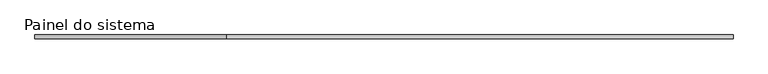
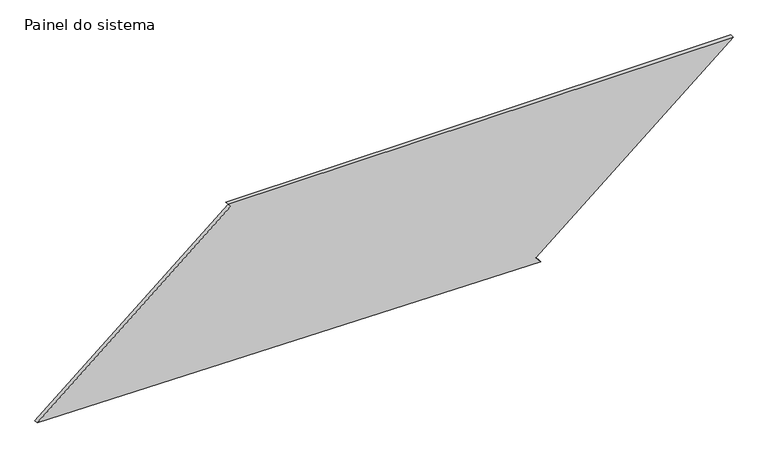
"""IFC4 building model written with IfcOpenShell, lengths in millimetres: plate geometry, Painel do sistema : Envidraçado."""

import ifcopenshell
import ifcopenshell.guid

model = None  # the IFC model being written
_history = None  # IfcOwnerHistory: only IFC2X3 demands one
_inside = {}  # id of a spatial element -> (the spatial element, [elements in it])
_under = {}  # id of a project, library or spatial element -> (it, [spatial elements below it])
_declared = {}  # id of a project -> (the project, [libraries it declares])
_typed = {}  # id of a type object -> (the type object, [elements of that type])
_made_of = {}  # id of a material, layer set ... -> (it, [elements and type objects made of it])


def new_model(schema):
    """Start an empty IFC model of exactly this schema.

    Asked for "IFC4X3", IfcOpenShell would pick the latest addendum, in which some entities
    have other attributes; the version numbers below select the first issue.
    IFC2X3 requires an IfcOwnerHistory on every rooted entity: one is made here for all.
    """
    global model, _history
    if schema == "IFC4X3":
        model = ifcopenshell.file(schema_version=(4, 3, 0, 0))
    else:
        model = ifcopenshell.file(schema=schema)
    _inside.clear()
    _under.clear()
    _declared.clear()
    _typed.clear()
    _made_of.clear()
    _history = None
    if model.schema == "IFC2X3":
        org = make("IfcOrganization", Name="unknown")
        user = make(
            "IfcPersonAndOrganization",
            ThePerson=make("IfcPerson", FamilyName="unknown"),
            TheOrganization=org,
        )
        app = make(
            "IfcApplication",
            ApplicationDeveloper=org,
            Version="unknown",
            ApplicationFullName="unknown",
            ApplicationIdentifier="unknown",
        )
        _history = make(
            "IfcOwnerHistory",
            OwningUser=user,
            OwningApplication=app,
            ChangeAction="ADDED",
            CreationDate=0,
        )
    return model


def make(cls, **values):
    """One entity of the class cls with the attributes given. An attribute that is None is left unset."""
    return model.create_entity(
        cls, **{name: value for name, value in values.items() if value is not None}
    )


def rooted(cls, **values):
    """An entity with a GlobalId (a new one), such as an element, a storey or a relation."""
    return make(cls, GlobalId=ifcopenshell.guid.new(), OwnerHistory=_history, **values)


def si_unit(unit_type, name, prefix=None):
    """IfcSIUnit, for example si_unit("LENGTHUNIT", "METRE", prefix="MILLI")."""
    return make("IfcSIUnit", UnitType=unit_type, Prefix=prefix, Name=name)


def assignment(units):
    """IfcUnitAssignment: the units of a project."""
    return None if units is None else make("IfcUnitAssignment", Units=units)


def point(xyz):
    """IfcCartesianPoint."""
    return None if xyz is None else make("IfcCartesianPoint", Coordinates=xyz)


def direction(xyz):
    """IfcDirection."""
    return None if xyz is None else make("IfcDirection", DirectionRatios=xyz)


def frame(location, z_axis=None, x_axis=None):
    """IfcAxis2Placement3D, a coordinate frame: its origin and axes. An axis left out is left unset."""
    return make(
        "IfcAxis2Placement3D",
        Location=point(location),
        Axis=direction(z_axis),
        RefDirection=direction(x_axis),
    )


def origin():
    """The frame at (0, 0, 0) with its axes left unset."""
    return frame((0.0, 0.0, 0.0))


def place(relative_to, where):
    """IfcLocalPlacement: puts the frame where relative to a parent placement (None: the world)."""
    return make(
        "IfcLocalPlacement", PlacementRelTo=relative_to, RelativePlacement=where
    )


def context(
    kind, dimensions, precision=None, world=None, true_north=None, identifier=None
):
    """IfcGeometricRepresentationContext, for example the 3D "Model" context."""
    return make(
        "IfcGeometricRepresentationContext",
        ContextIdentifier=identifier,
        ContextType=kind,
        CoordinateSpaceDimension=dimensions,
        Precision=precision,
        WorldCoordinateSystem=world,
        TrueNorth=true_north,
    )


def project(units=None, contexts=None):
    """IfcProject with its units and contexts."""
    return rooted(
        "IfcProject",
        Name="project",
        RepresentationContexts=contexts,
        UnitsInContext=assignment(units),
    )


def spatial(cls, under=None, at=None, **own):
    """A site, building, storey or space (cls), placed at a placement, below another one or the project."""
    s = rooted(cls, ObjectPlacement=at, **own)
    if under is not None:
        _under.setdefault(under.id(), (under, []))[1].append(s)
    return s


def polyline(points):
    """IfcPolyline through the points."""
    return make("IfcPolyline", Points=[point(p) for p in points])


def outline(outer, holes=None, kind="AREA"):
    """IfcArbitraryClosedProfileDef: a profile drawn as a closed curve; with holes, ...WithVoids."""
    if holes is None:
        return make("IfcArbitraryClosedProfileDef", ProfileType=kind, OuterCurve=outer)
    return make(
        "IfcArbitraryProfileDefWithVoids",
        ProfileType=kind,
        OuterCurve=outer,
        InnerCurves=holes,
    )


def extrude(swept, where, along, depth):
    """IfcExtrudedAreaSolid: the profile swept, set in the frame where, extruded along a direction by depth."""
    return make(
        "IfcExtrudedAreaSolid",
        SweptArea=swept,
        Position=where,
        ExtrudedDirection=direction(along),
        Depth=depth,
    )


def shape(context_of_items, identifier, shape_type, items):
    """IfcShapeRepresentation: the items that make up one representation, for example the "Body"."""
    return make(
        "IfcShapeRepresentation",
        ContextOfItems=context_of_items,
        RepresentationIdentifier=identifier,
        RepresentationType=shape_type,
        Items=items,
    )


def source(mapping_origin, context_of_items, identifier, shape_type, items):
    """IfcRepresentationMap: a shape defined once, which mapped items show again and again."""
    return make(
        "IfcRepresentationMap",
        MappingOrigin=mapping_origin,
        MappedRepresentation=shape(context_of_items, identifier, shape_type, items),
    )


def transform(
    local_origin,
    x_axis=None,
    y_axis=None,
    z_axis=None,
    scale=None,
    scale2=None,
    scale3=None,
    uniform=True,
):
    """IfcCartesianTransformationOperator3D, or its non-uniform kind. x_axis, y_axis, z_axis: its Axis1, 2, 3."""
    if uniform:
        return make(
            "IfcCartesianTransformationOperator3D",
            Axis1=direction(x_axis),
            Axis2=direction(y_axis),
            LocalOrigin=point(local_origin),
            Scale=scale,
            Axis3=direction(z_axis),
        )
    return make(
        "IfcCartesianTransformationOperator3DnonUniform",
        Axis1=direction(x_axis),
        Axis2=direction(y_axis),
        LocalOrigin=point(local_origin),
        Scale=scale,
        Axis3=direction(z_axis),
        Scale2=scale2,
        Scale3=scale3,
    )


def mapped(mapping_source, mapping_target):
    """IfcMappedItem: shows the shape of a source again, moved by a transform."""
    return make(
        "IfcMappedItem", MappingSource=mapping_source, MappingTarget=mapping_target
    )


def made_of(thing, what):
    """Note that an element or type object is made of a material, layer set ...; save() writes the relation."""
    if what is not None:
        _made_of.setdefault(what.id(), (what, []))[1].append(thing)
    return thing


def element(
    cls,
    number,
    at=None,
    inside=None,
    cuts=None,
    type_object=None,
    material=None,
    context=None,
    identifier="Body",
    shape_type=None,
    held_by="IfcProductDefinitionShape",
    body=None,
    shapes=None,
    **own,
):
    """One element of the class cls, such as IfcWall. Its Tag is "e" and its number.

    at: its placement. inside: the storey or other place that contains it. cuts: it is an
    opening in that element (IfcRelVoidsElement). A single representation is given by context,
    identifier, shape_type and body (its items); several are given by shapes. held_by: the class
    of the entity that holds the representations. save() writes the other relations.
    """
    e = rooted(cls, Tag="e%d" % number, ObjectPlacement=at, **own)
    if body is not None:
        shapes = [shape(context, identifier, shape_type, body)]
    if shapes is not None:
        e.Representation = make(held_by, Representations=shapes)
    if inside is not None:
        _inside.setdefault(inside.id(), (inside, []))[1].append(e)
    if cuts is not None:
        rooted(
            "IfcRelVoidsElement", RelatingBuildingElement=cuts, RelatedOpeningElement=e
        )
    if type_object is not None:
        _typed.setdefault(type_object.id(), (type_object, []))[1].append(e)
    return made_of(e, material)


def aggregate(whole, parts):
    """IfcRelAggregates: a whole, such as a stair, and the parts it consists of."""
    return rooted("IfcRelAggregates", RelatingObject=whole, RelatedObjects=parts)


def save(model, path):
    """Write the relations noted so far, then the file.

    IfcRelAggregates (storeys below a building ...), IfcRelContainedInSpatialStructure (elements
    in a storey), IfcRelDefinesByType, IfcRelAssociatesMaterial and IfcRelDeclares: one each for
    every whole, place, type object, material and project.
    """
    for whole, parts in _under.values():
        aggregate(whole, parts)
    for where, things in _inside.values():
        rooted(
            "IfcRelContainedInSpatialStructure",
            RelatedElements=things,
            RelatingStructure=where,
        )
    for kind, things in _typed.values():
        rooted("IfcRelDefinesByType", RelatedObjects=things, RelatingType=kind)
    for what, things in _made_of.values():
        rooted("IfcRelAssociatesMaterial", RelatedObjects=things, RelatingMaterial=what)
    for by, libraries in _declared.values():
        rooted("IfcRelDeclares", RelatingContext=by, RelatedDefinitions=libraries)
    model.write(path)


def painel_do_sistema_b8f4bcb4(model_context):
    return source(origin(), model_context, "Body", "SweptSolid", [
        extrude(outline(polyline([(0.0, 1005.4581912), (38.4075918, 973.444805), (1099.1556087, 2246.0617236), (1099.1556087, -1013.2862331), (1079.9518128, -997.27954), (39.0704561, -2246.0617236), (0.0, 1005.4581912)])), frame((0.0, 24.5, 0.0), z_axis=(0.0, 1.0, 0.0), x_axis=(0.0, 0.0, 1.0)), (0.0, 0.0, 1.0), 25.0),
    ])


if __name__ == "__main__":
    model = new_model("IFC4")
    model_context = context("Model", 3, world=origin())
    ifc_project = project(units=[si_unit("LENGTHUNIT", "METRE", prefix="MILLI")], contexts=[model_context])
    site = spatial("IfcSite", under=ifc_project)
    building = spatial("IfcBuilding", under=site)
    placement = place(None, origin())
    painel_do_sistema_shape = painel_do_sistema_b8f4bcb4(model_context)
    element("IfcPlate", 1, ObjectType="Painel do sistema : Envidraçado", at=placement, inside=building, context=model_context, shape_type="MappedRepresentation", body=[
        mapped(painel_do_sistema_shape, transform((0.0, 0.0, 0.0), x_axis=(1.0, 0.0, 0.0), y_axis=(0.0, 1.0, 0.0), z_axis=(0.0, 0.0, 1.0))),
    ])
    save(model, "model.ifc")

# Revit data of these elements
# Type "Painel do sistema : Envidraçado"
#   Construction Type Id = "GSP4R"
#   Analytic Construction = "Vidraça única Pilkington 1/8 pol"
#   Visual Light Transmittance = 0.9
#   Solar Heat Gain Coefficient = 0.86
#   Heat Transfer Coefficient (U) = 6.7069 W/(m²·K)
# Element 1 (IfcPlate, "Painel do sistema : Envidraçado")
#   Materials on its faces: "Vidro"
# Materials
#   "Vidro": class "Vidro", colour RGB 0 128 192, transparency 0.9, Description = "Vidro de sílica", Cost = 0
